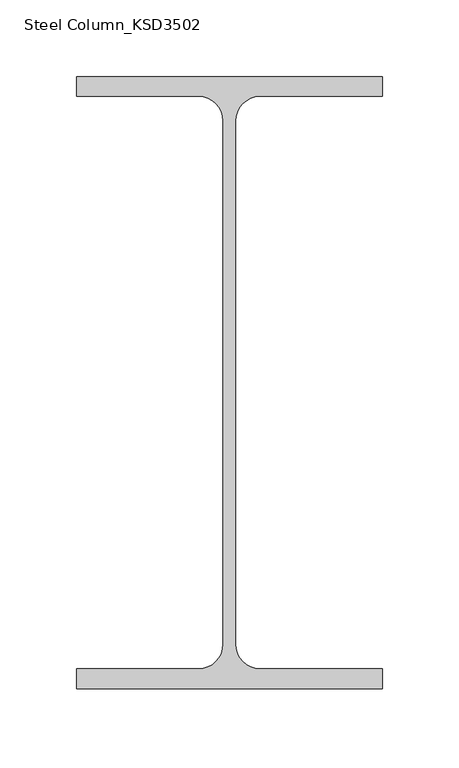
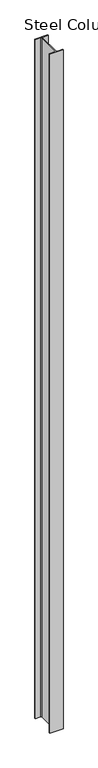
"""IFC4 building model written with IfcOpenShell, lengths in millimetres: column geometry, Steel Column_KSD3502 : H_SC_ASC_H-400×200x8x13."""

from ifc_helpers import new_model, si_unit, point, frame, frame_2d, origin, place, context, project, spatial, polyline, circle_curve, trimmed, segment, composite_curve, outline, extrude, source, transform, mapped, element, save


def steel_column_ksd3502_1d3624df(model_context):
    return source(origin(), model_context, "Body", "SweptSolid", [
        extrude(outline(composite_curve([segment(polyline([(100.0, 200.0), (100.0, 187.0), (20.0, 187.0)]), True, "CONTINUOUS"), segment(trimmed(circle_curve(frame_2d((20.0, 171.0)), 16.0), [point((20.0, 187.0))], [point((4.0, 171.0))], True, "CARTESIAN"), True, "CONTINUOUS"), segment(polyline([(4.0, 171.0), (4.0, -171.0)]), True, "CONTINUOUS"), segment(trimmed(circle_curve(frame_2d((20.0, -171.0)), 16.0), [point((4.0, -171.0))], [point((20.0, -187.0))], True, "CARTESIAN"), True, "CONTINUOUS"), segment(polyline([(20.0, -187.0), (100.0, -187.0), (100.0, -200.0), (-100.0, -200.0), (-100.0, -187.0), (-20.0, -187.0)]), True, "CONTINUOUS"), segment(trimmed(circle_curve(frame_2d((-20.0, -171.0)), 16.0), [point((-20.0, -187.0))], [point((-4.0, -171.0))], True, "CARTESIAN"), True, "CONTINUOUS"), segment(polyline([(-4.0, -171.0), (-4.0, 171.0)]), True, "CONTINUOUS"), segment(trimmed(circle_curve(frame_2d((-20.0, 171.0)), 16.0), [point((-4.0, 171.0))], [point((-20.0, 187.0))], True, "CARTESIAN"), True, "CONTINUOUS"), segment(polyline([(-20.0, 187.0), (-100.0, 187.0), (-100.0, 200.0), (100.0, 200.0)]), True, "CONTINUOUS")], self_intersect=False)), frame((0.0, 0.0, 6949.9720055), z_axis=(0.0, 0.0, 1.0), x_axis=(1.0, 0.0, 0.0)), (0.0, 0.0, 1.0), 11000.0),
    ])


if __name__ == "__main__":
    model = new_model("IFC4")
    model_context = context("Model", 3, world=origin())
    ifc_project = project(units=[si_unit("LENGTHUNIT", "METRE", prefix="MILLI")], contexts=[model_context])
    site = spatial("IfcSite", under=ifc_project)
    building = spatial("IfcBuilding", under=site)
    placement = place(None, origin())
    steel_column_ksd3502_shape = steel_column_ksd3502_1d3624df(model_context)
    element("IfcColumn", 1, ObjectType="Steel Column_KSD3502 : H_SC_ASC_H-400×200x8x13", at=placement, inside=building, context=model_context, shape_type="MappedRepresentation", body=[
        mapped(steel_column_ksd3502_shape, transform((0.0, 0.0, 0.0), x_axis=(1.0, 0.0, 0.0), y_axis=(0.0, 1.0, 0.0), z_axis=(0.0, 0.0, 1.0))),
    ])
    save(model, "model.ifc")

# Revit data of these elements
# Type "Steel Column_KSD3502 : H_SC_ASC_H-400×200x8x13"
#   Width = 20.0 cm
#   Web Thickness = 0.8 cm
#   Web Fillet = 1.6 cm
#   Warping Constant = 648999.0 cm⁶
#   Torsional Moment of Inertia = 35.8981 cm⁴
#   Section Area = 84.12 cm²
#   Plastic Modulus weak axis = 268.0 cm³
#   Plastic Modulus strong axis = 1330.0 cm³
#   Perimeter = 1.27 m²/m
#   Nominal Weight = 66.00 kgf/m
#   Moment of Inertia weak axis = 1740.00 cm⁴
#   Moment of Inertia strong axis = 23700.00 cm⁴
#   Height = 40.0 cm
#   Flange Thickness = 1.3 cm
#   Elastic Modulus weak axis = 174.0 cm³
#   Elastic Modulus strong axis = 1190.0 cm³
#   Centroid Vertical = 20.0 cm
#   Centroid Horizontal = 10.0 cm
#   Bolt Spacing = 13.97 cm
#   Structural Material [instance default] = Steel, 45-345
#   Section Name Key = ""
#   Assembly Code = ""
# Element 1 (IfcColumn, "Steel Column_KSD3502 : H_SC_ASC_H-400×200x8x13")
#   Structural Material = none
# Materials
#   "Steel, 45-345": class "Metal", colour RGB 189 187 185, transparency 0, Description = "Steel 345 MPa", Cost = 0
